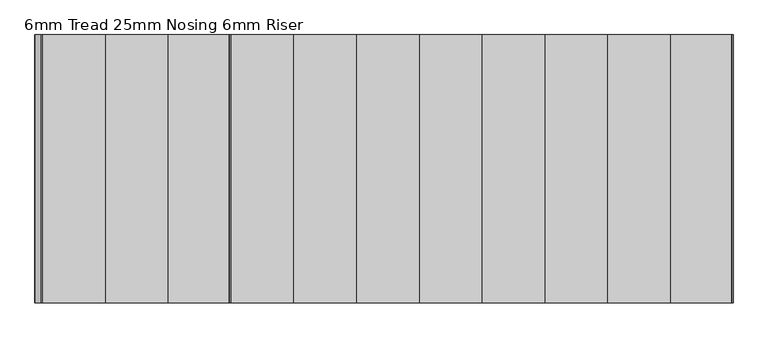
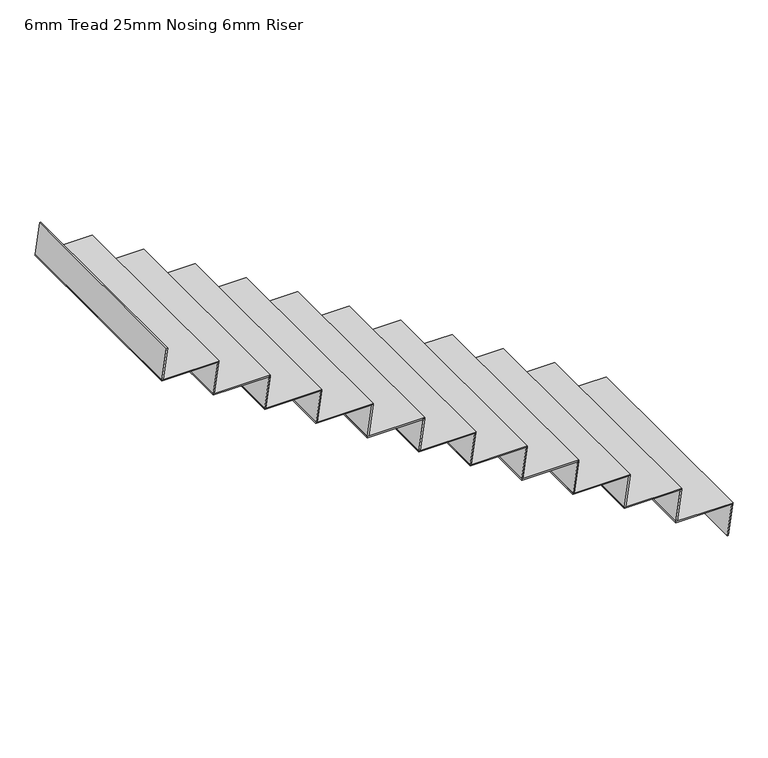
"""IFC4 building model written with IfcOpenShell, lengths in millimetres: stair flight geometry, 6mm Tread 25mm Nosing 6mm Riser."""

from ifc_helpers import new_model, si_unit, origin, place, context, project, spatial, faceted_brep, source, transform, mapped, element, save


def stair_flight_6mm_tread_25mm_nosing_6mm_riser_063e3d0e(model_context):
    return source(origin(), model_context, "Body", "Brep", [
        faceted_brep([(-13631.0599092, 11395.4345331, 28647.0588235), (-13631.9099092, 11395.4345331, 28641.0588235), (-13631.9099092, 10220.4345331, 28641.0588235), (-13631.0599092, 10220.4345331, 28647.0588235), (-13325.0, 10220.4345331, 28647.0588235), (-13325.0, 11395.4345331, 28647.0588235), (-13325.85, 11395.4345331, 28641.0588235), (-13325.85, 10220.4345331, 28641.0588235)], [[[0, 1, 2, 3]], [[3, 4, 5, 0]], [[2, 1, 6, 7]], [[4, 3, 2, 7]], [[0, 5, 6, 1]], [[5, 4, 7, 6]]]),
        faceted_brep([(-13325.85, 11395.4345331, 28641.0588235), (-13350.0, 11395.4345331, 28470.5882353), (-13356.0599092, 11395.4345331, 28470.5882353), (-13331.9099092, 11395.4345331, 28641.0588235), (-13325.85, 10220.4345331, 28641.0588235), (-13331.9099092, 10220.4345331, 28641.0588235), (-13356.0599092, 10220.4345331, 28470.5882353), (-13350.0, 10220.4345331, 28470.5882353)], [[[0, 1, 2, 3]], [[4, 5, 6, 7]], [[1, 0, 4, 7]], [[2, 1, 7, 6]], [[3, 2, 6, 5]], [[0, 3, 5, 4]]]),
        faceted_brep([(-13600.85, 11395.4345331, 28817.5294118), (-13625.0, 11395.4345331, 28647.0588235), (-13631.0599092, 11395.4345331, 28647.0588235), (-13606.9099092, 11395.4345331, 28817.5294118), (-13600.85, 10220.4345331, 28817.5294118), (-13606.9099092, 10220.4345331, 28817.5294118), (-13631.0599092, 10220.4345331, 28647.0588235), (-13625.0, 10220.4345331, 28647.0588235)], [[[0, 1, 2, 3]], [[4, 5, 6, 7]], [[1, 0, 4, 7]], [[2, 1, 7, 6]], [[3, 2, 6, 5]], [[0, 3, 5, 4]]]),
        faceted_brep([(-13906.0599092, 10220.4345331, 28823.5294118), (-13600.0, 10220.4345331, 28823.5294118), (-13600.0, 11395.4345331, 28823.5294118), (-13906.0599092, 11395.4345331, 28823.5294118), (-13906.9099092, 10220.4345331, 28817.5294118), (-13906.9099092, 11395.4345331, 28817.5294118), (-13600.85, 11395.4345331, 28817.5294118), (-13600.85, 10220.4345331, 28817.5294118)], [[[0, 1, 2, 3]], [[4, 5, 6, 7]], [[1, 0, 4, 7]], [[3, 2, 6, 5]], [[3, 5, 4, 0]], [[2, 1, 7, 6]]]),
        faceted_brep([(-13875.85, 11395.4345331, 28994.0), (-13900.0, 11395.4345331, 28823.5294118), (-13906.0599092, 11395.4345331, 28823.5294118), (-13881.9099092, 11395.4345331, 28994.0), (-13875.85, 10220.4345331, 28994.0), (-13881.9099092, 10220.4345331, 28994.0), (-13906.0599092, 10220.4345331, 28823.5294118), (-13900.0, 10220.4345331, 28823.5294118)], [[[0, 1, 2, 3]], [[4, 5, 6, 7]], [[1, 0, 4, 7]], [[2, 1, 7, 6]], [[3, 2, 6, 5]], [[0, 3, 5, 4]]]),
        faceted_brep([(-14181.0599092, 10220.4345331, 29000.0), (-13875.0, 10220.4345331, 29000.0), (-13875.0, 11395.4345331, 29000.0), (-14181.0599092, 11395.4345331, 29000.0), (-14181.9099092, 10220.4345331, 28994.0), (-14181.9099092, 11395.4345331, 28994.0), (-13875.85, 11395.4345331, 28994.0), (-13875.85, 10220.4345331, 28994.0)], [[[0, 1, 2, 3]], [[4, 5, 6, 7]], [[1, 0, 4, 7]], [[3, 2, 6, 5]], [[3, 5, 4, 0]], [[2, 1, 7, 6]]]),
        faceted_brep([(-14150.85, 11395.4345331, 29170.4705882), (-14175.0, 11395.4345331, 29000.0), (-14181.0599092, 11395.4345331, 29000.0), (-14156.9099092, 11395.4345331, 29170.4705882), (-14150.85, 10220.4345331, 29170.4705882), (-14156.9099092, 10220.4345331, 29170.4705882), (-14181.0599092, 10220.4345331, 29000.0), (-14175.0, 10220.4345331, 29000.0)], [[[0, 1, 2, 3]], [[4, 5, 6, 7]], [[1, 0, 4, 7]], [[2, 1, 7, 6]], [[3, 2, 6, 5]], [[0, 3, 5, 4]]]),
        faceted_brep([(-14456.0599092, 10220.4345331, 29176.4705882), (-14150.0, 10220.4345331, 29176.4705882), (-14150.0, 11395.4345331, 29176.4705882), (-14456.0599092, 11395.4345331, 29176.4705882), (-14456.9099092, 10220.4345331, 29170.4705882), (-14456.9099092, 11395.4345331, 29170.4705882), (-14150.85, 11395.4345331, 29170.4705882), (-14150.85, 10220.4345331, 29170.4705882)], [[[0, 1, 2, 3]], [[4, 5, 6, 7]], [[1, 0, 4, 7]], [[3, 2, 6, 5]], [[3, 5, 4, 0]], [[2, 1, 7, 6]]]),
        faceted_brep([(-14425.85, 11395.4345331, 29346.9411765), (-14450.0, 11395.4345331, 29176.4705882), (-14456.0599092, 11395.4345331, 29176.4705882), (-14431.9099092, 11395.4345331, 29346.9411765), (-14425.85, 10220.4345331, 29346.9411765), (-14431.9099092, 10220.4345331, 29346.9411765), (-14456.0599092, 10220.4345331, 29176.4705882), (-14450.0, 10220.4345331, 29176.4705882)], [[[0, 1, 2, 3]], [[4, 5, 6, 7]], [[1, 0, 4, 7]], [[2, 1, 7, 6]], [[3, 2, 6, 5]], [[0, 3, 5, 4]]]),
        faceted_brep([(-14731.0599092, 10220.4345331, 29352.9411765), (-14425.0, 10220.4345331, 29352.9411765), (-14425.0, 11395.4345331, 29352.9411765), (-14731.0599092, 11395.4345331, 29352.9411765), (-14731.9099092, 10220.4345331, 29346.9411765), (-14731.9099092, 11395.4345331, 29346.9411765), (-14425.85, 11395.4345331, 29346.9411765), (-14425.85, 10220.4345331, 29346.9411765)], [[[0, 1, 2, 3]], [[4, 5, 6, 7]], [[1, 0, 4, 7]], [[3, 2, 6, 5]], [[3, 5, 4, 0]], [[2, 1, 7, 6]]]),
        faceted_brep([(-14700.85, 11395.4345331, 29523.4117647), (-14725.0, 11395.4345331, 29352.9411765), (-14731.0599092, 11395.4345331, 29352.9411765), (-14706.9099092, 11395.4345331, 29523.4117647), (-14700.85, 10220.4345331, 29523.4117647), (-14706.9099092, 10220.4345331, 29523.4117647), (-14731.0599092, 10220.4345331, 29352.9411765), (-14725.0, 10220.4345331, 29352.9411765)], [[[0, 1, 2, 3]], [[4, 5, 6, 7]], [[1, 0, 4, 7]], [[2, 1, 7, 6]], [[3, 2, 6, 5]], [[0, 3, 5, 4]]]),
        faceted_brep([(-15006.0599092, 10220.4345331, 29529.4117647), (-14700.0, 10220.4345331, 29529.4117647), (-14700.0, 11395.4345331, 29529.4117647), (-15006.0599092, 11395.4345331, 29529.4117647), (-15006.9099092, 10220.4345331, 29523.4117647), (-15006.9099092, 11395.4345331, 29523.4117647), (-14700.85, 11395.4345331, 29523.4117647), (-14700.85, 10220.4345331, 29523.4117647)], [[[0, 1, 2, 3]], [[4, 5, 6, 7]], [[1, 0, 4, 7]], [[3, 2, 6, 5]], [[3, 5, 4, 0]], [[2, 1, 7, 6]]]),
        faceted_brep([(-14975.85, 11395.4345331, 29699.8823529), (-15000.0, 11395.4345331, 29529.4117647), (-15006.0599092, 11395.4345331, 29529.4117647), (-14981.9099092, 11395.4345331, 29699.8823529), (-14975.85, 10220.4345331, 29699.8823529), (-14981.9099092, 10220.4345331, 29699.8823529), (-15006.0599092, 10220.4345331, 29529.4117647), (-15000.0, 10220.4345331, 29529.4117647)], [[[0, 1, 2, 3]], [[4, 5, 6, 7]], [[1, 0, 4, 7]], [[2, 1, 7, 6]], [[3, 2, 6, 5]], [[0, 3, 5, 4]]]),
        faceted_brep([(-15281.0599092, 10220.4345331, 29705.8823529), (-14975.0, 10220.4345331, 29705.8823529), (-14975.0, 11395.4345331, 29705.8823529), (-15281.0599092, 11395.4345331, 29705.8823529), (-15281.9099092, 10220.4345331, 29699.8823529), (-15281.9099092, 11395.4345331, 29699.8823529), (-14975.85, 11395.4345331, 29699.8823529), (-14975.85, 10220.4345331, 29699.8823529)], [[[0, 1, 2, 3]], [[4, 5, 6, 7]], [[1, 0, 4, 7]], [[3, 2, 6, 5]], [[3, 5, 4, 0]], [[2, 1, 7, 6]]]),
        faceted_brep([(-15250.85, 11395.4345331, 29876.3529412), (-15275.0, 11395.4345331, 29705.8823529), (-15281.0599092, 11395.4345331, 29705.8823529), (-15256.9099092, 11395.4345331, 29876.3529412), (-15250.85, 10220.4345331, 29876.3529412), (-15256.9099092, 10220.4345331, 29876.3529412), (-15281.0599092, 10220.4345331, 29705.8823529), (-15275.0, 10220.4345331, 29705.8823529)], [[[0, 1, 2, 3]], [[4, 5, 6, 7]], [[1, 0, 4, 7]], [[2, 1, 7, 6]], [[3, 2, 6, 5]], [[0, 3, 5, 4]]]),
        faceted_brep([(-15556.0599092, 10220.4345331, 29882.3529412), (-15250.0, 10220.4345331, 29882.3529412), (-15250.0, 11395.4345331, 29882.3529412), (-15556.0599092, 11395.4345331, 29882.3529412), (-15556.9099092, 10220.4345331, 29876.3529412), (-15556.9099092, 11395.4345331, 29876.3529412), (-15250.85, 11395.4345331, 29876.3529412), (-15250.85, 10220.4345331, 29876.3529412)], [[[0, 1, 2, 3]], [[4, 5, 6, 7]], [[1, 0, 4, 7]], [[3, 2, 6, 5]], [[3, 5, 4, 0]], [[2, 1, 7, 6]]]),
        faceted_brep([(-15525.85, 11395.4345331, 30052.8235294), (-15550.0, 11395.4345331, 29882.3529412), (-15556.0599092, 11395.4345331, 29882.3529412), (-15531.9099092, 11395.4345331, 30052.8235294), (-15525.85, 10220.4345331, 30052.8235294), (-15531.9099092, 10220.4345331, 30052.8235294), (-15556.0599092, 10220.4345331, 29882.3529412), (-15550.0, 10220.4345331, 29882.3529412)], [[[0, 1, 2, 3]], [[4, 5, 6, 7]], [[1, 0, 4, 7]], [[2, 1, 7, 6]], [[3, 2, 6, 5]], [[0, 3, 5, 4]]]),
        faceted_brep([(-15831.0599092, 10220.4345331, 30058.8235294), (-15525.0, 10220.4345331, 30058.8235294), (-15525.0, 11395.4345331, 30058.8235294), (-15831.0599092, 11395.4345331, 30058.8235294), (-15831.9099092, 10220.4345331, 30052.8235294), (-15831.9099092, 11395.4345331, 30052.8235294), (-15525.85, 11395.4345331, 30052.8235294), (-15525.85, 10220.4345331, 30052.8235294)], [[[0, 1, 2, 3]], [[4, 5, 6, 7]], [[1, 0, 4, 7]], [[3, 2, 6, 5]], [[3, 5, 4, 0]], [[2, 1, 7, 6]]]),
        faceted_brep([(-15800.85, 11395.4345331, 30229.2941176), (-15825.0, 11395.4345331, 30058.8235294), (-15831.0599092, 11395.4345331, 30058.8235294), (-15806.9099092, 11395.4345331, 30229.2941176), (-15800.85, 10220.4345331, 30229.2941176), (-15806.9099092, 10220.4345331, 30229.2941176), (-15831.0599092, 10220.4345331, 30058.8235294), (-15825.0, 10220.4345331, 30058.8235294)], [[[0, 1, 2, 3]], [[4, 5, 6, 7]], [[1, 0, 4, 7]], [[2, 1, 7, 6]], [[3, 2, 6, 5]], [[0, 3, 5, 4]]]),
        faceted_brep([(-16106.0599092, 10220.4345331, 30235.2941176), (-15800.0, 10220.4345331, 30235.2941176), (-15800.0, 11395.4345331, 30235.2941176), (-16106.0599092, 11395.4345331, 30235.2941176), (-16106.9099092, 10220.4345331, 30229.2941176), (-16106.9099092, 11395.4345331, 30229.2941176), (-15800.85, 11395.4345331, 30229.2941176), (-15800.85, 10220.4345331, 30229.2941176)], [[[0, 1, 2, 3]], [[4, 5, 6, 7]], [[1, 0, 4, 7]], [[3, 2, 6, 5]], [[3, 5, 4, 0]], [[2, 1, 7, 6]]]),
        faceted_brep([(-16350.85, 11395.4345331, 30582.2352941), (-16375.0, 11395.4345331, 30411.7647059), (-16381.0599092, 11395.4345331, 30411.7647059), (-16356.9099092, 11395.4345331, 30582.2352941), (-16350.85, 10220.4345331, 30582.2352941), (-16356.9099092, 10220.4345331, 30582.2352941), (-16381.0599092, 10220.4345331, 30411.7647059), (-16375.0, 10220.4345331, 30411.7647059)], [[[0, 1, 2, 3]], [[4, 5, 6, 7]], [[1, 0, 4, 7]], [[2, 1, 7, 6]], [[3, 2, 6, 5]], [[0, 3, 5, 4]]]),
        faceted_brep([(-16075.85, 11395.4345331, 30405.7647059), (-16100.0, 11395.4345331, 30235.2941176), (-16106.0599092, 11395.4345331, 30235.2941176), (-16081.9099092, 11395.4345331, 30405.7647059), (-16075.85, 10220.4345331, 30405.7647059), (-16081.9099092, 10220.4345331, 30405.7647059), (-16106.0599092, 10220.4345331, 30235.2941176), (-16100.0, 10220.4345331, 30235.2941176)], [[[0, 1, 2, 3]], [[4, 5, 6, 7]], [[1, 0, 4, 7]], [[2, 1, 7, 6]], [[3, 2, 6, 5]], [[0, 3, 5, 4]]]),
        faceted_brep([(-16381.0599092, 10220.4345331, 30411.7647059), (-16350.0, 10220.4345331, 30411.7647059), (-16075.0, 10220.4345331, 30411.7647059), (-16075.0, 11395.4345331, 30411.7647059), (-16381.0599092, 11395.4345331, 30411.7647059), (-16381.9099092, 10220.4345331, 30405.7647059), (-16381.9099092, 11395.4345331, 30405.7647059), (-16075.85, 11395.4345331, 30405.7647059), (-16075.85, 10220.4345331, 30405.7647059), (-16350.0, 10220.4345331, 30405.7647059)], [[[0, 1, 2, 3, 4]], [[5, 6, 7, 8, 9]], [[1, 0, 5, 9]], [[2, 1, 9, 8]], [[4, 3, 7, 6]], [[4, 6, 5, 0]], [[3, 2, 8, 7]]]),
    ])


if __name__ == "__main__":
    model = new_model("IFC4")
    model_context = context("Model", 3, world=origin())
    ifc_project = project(units=[si_unit("LENGTHUNIT", "METRE", prefix="MILLI")], contexts=[model_context])
    site = spatial("IfcSite", under=ifc_project)
    building = spatial("IfcBuilding", under=site)
    placement = place(None, origin())
    stair_flight_6mm_tread_25mm_nosing_6mm_riser_shape = stair_flight_6mm_tread_25mm_nosing_6mm_riser_063e3d0e(model_context)
    element("IfcStairFlight", 1, ObjectType="6mm Tread 25mm Nosing 6mm Riser", at=placement, inside=building, context=model_context, shape_type="MappedRepresentation", body=[
        mapped(stair_flight_6mm_tread_25mm_nosing_6mm_riser_shape, transform((0.0, 0.0, 0.0), x_axis=(1.0, 0.0, 0.0), y_axis=(0.0, 1.0, 0.0), z_axis=(0.0, 0.0, 1.0))),
    ])
    save(model, "model.ifc")

# Revit data of these elements
# Element 1 (IfcStairFlight, "6mm Tread 25mm Nosing 6mm Riser")
#   Materials on its faces: "Steel, Paint Finish, Dark Gray"
# Materials
#   "Steel, Paint Finish, Dark Gray": class "Metal", colour RGB 89 89 89, transparency 0, Description = "Steel, paint finish, dark gray, glossy", Cost = 0
